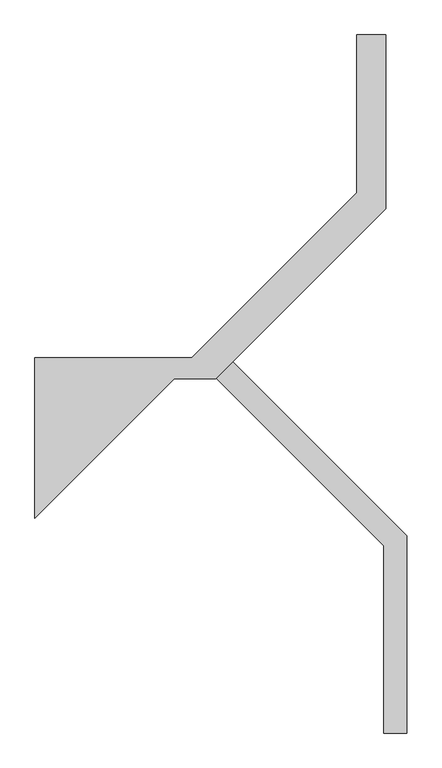
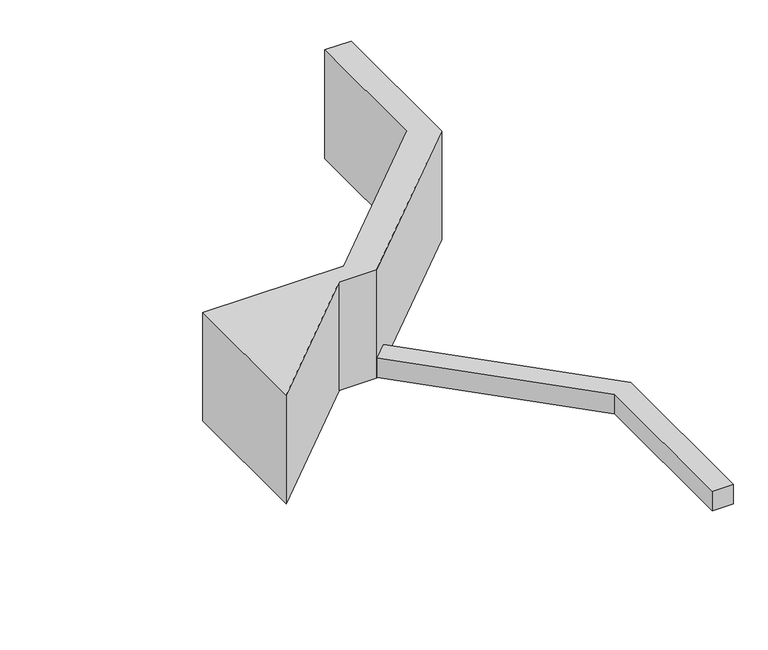
"""IFC4 building model written with IfcOpenShell, lengths in millimetres: furniture geometry, Master Bath shower & tub base : Master Bath shower & tub base."""

from ifc_helpers import new_model, si_unit, origin, origin_with_axes, place, context, project, spatial, polyline, outline, extrude, source, transform, mapped, element, save


def furniture_67438e5e(model_context):
    return source(origin(), model_context, "Body", "SweptSolid", [
        extrude(outline(polyline([(-9442.45, 14236.7), (-9625.1994265, 14236.7), (-10234.7994265, 13627.1), (-10234.7994265, 14328.6414107), (-9548.9789473, 14328.6414107), (-8825.6599552, 15051.9604028), (-8825.6599552, 15743.2375), (-8697.9125, 15743.2375), (-8697.9125, 14981.2375), (-9442.45, 14236.7)])), origin_with_axes(), (0.0, 0.0, 1.0), 558.8),
        extrude(outline(polyline([(-8605.8375, 12685.7125), (-8707.4375, 12685.7125), (-8707.4375, 13507.2284021), (-9439.679549, 14239.470451), (-9367.8375, 14311.3125), (-8605.8375, 13549.3125), (-8605.8375, 12685.7125)])), origin_with_axes(), (0.0, 0.0, 1.0), 101.6),
    ])


if __name__ == "__main__":
    model = new_model("IFC4")
    model_context = context("Model", 3, world=origin())
    ifc_project = project(units=[si_unit("LENGTHUNIT", "METRE", prefix="MILLI")], contexts=[model_context])
    site = spatial("IfcSite", under=ifc_project)
    building = spatial("IfcBuilding", under=site)
    placement = place(None, origin())
    furniture_shape = furniture_67438e5e(model_context)
    element("IfcFurniture", 1, ObjectType="Master Bath shower & tub base : Master Bath shower & tub base", at=placement, inside=building, context=model_context, shape_type="MappedRepresentation", body=[
        mapped(furniture_shape, transform((0.0, 0.0, 0.0), x_axis=(1.0, 0.0, 0.0), y_axis=(0.0, 1.0, 0.0), z_axis=(0.0, 0.0, 1.0))),
    ])
    save(model, "model.ifc")

# Revit data of these elements
# Type "Master Bath shower & tub base : Master Bath shower & tub base"
#   COBie.Type = no
# Element 1 (IfcFurniture, "Master Bath shower & tub base : Master Bath shower & tub base")
#   Materials on its faces: "Tile, grey Green"
# Materials
#   "Tile, grey Green": class "Generic", colour RGB 70 104 106, transparency 0, Description = "Porcelain tile, 4\", white", Cost = 0
